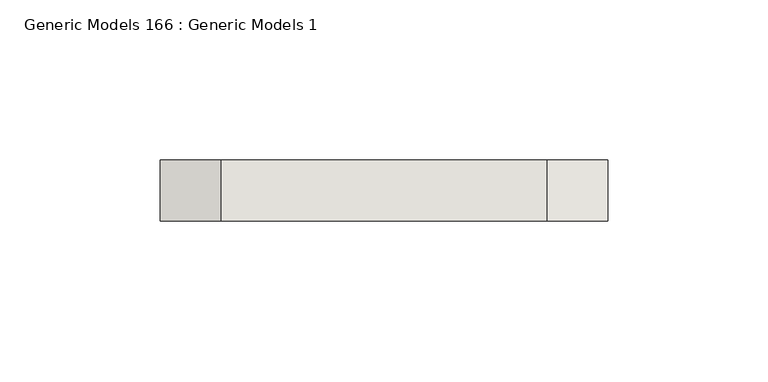
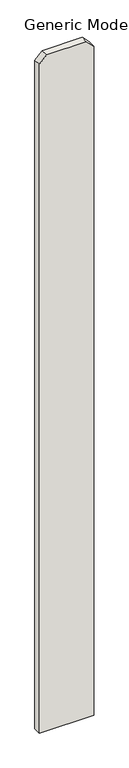
"""IFC4 building model written with IfcOpenShell, lengths in millimetres: wall geometry, Generic Models 166 : Generic Models 1."""

from ifc_helpers import new_model, si_unit, frame, origin, place, context, project, spatial, polyline, outline, extrude, source, transform, mapped, element, save


def generic_models_166_generic_models_1_02abbdc1(model_context):
    return source(origin(), model_context, "Body", "SweptSolid", [
        extrude(outline(polyline([(76.2, 324280.2125), (1885.95, 324280.2125), (1905.0, 324261.1625), (1905.0, 324159.5625), (1885.95, 324140.5125), (76.2, 324140.5125), (76.2, 324280.2125)])), frame((0.0, 547.6875, 0.0), z_axis=(0.0, 1.0, 0.0), x_axis=(0.0, 0.0, 1.0)), (0.0, 0.0, 1.0), 19.05),
    ])


if __name__ == "__main__":
    model = new_model("IFC4")
    model_context = context("Model", 3, world=origin())
    ifc_project = project(units=[si_unit("LENGTHUNIT", "METRE", prefix="MILLI")], contexts=[model_context])
    site = spatial("IfcSite", under=ifc_project)
    building = spatial("IfcBuilding", under=site)
    placement = place(None, origin())
    generic_models_166_generic_models_1_shape = generic_models_166_generic_models_1_02abbdc1(model_context)
    element("IfcWall", 1, ObjectType="Generic Models 166 : Generic Models 1", at=placement, inside=building, context=model_context, shape_type="MappedRepresentation", body=[
        mapped(generic_models_166_generic_models_1_shape, transform((0.0, 0.0, 0.0), x_axis=(1.0, 0.0, 0.0), y_axis=(0.0, 1.0, 0.0), z_axis=(0.0, 0.0, 1.0))),
    ])
    save(model, "model.ifc")

# Revit data of these elements
# Element 1 (IfcWall, "Generic Models 166 : Generic Models 1")
#   Materials on its faces: "VERTICAL 1X6 CEDAR PLANKS W/ CLEAR WOOD SEALER"
# Materials
#   "VERTICAL 1X6 CEDAR PLANKS W/ CLEAR WOOD SEALER": class "Wood", colour RGB 234 198 147, transparency 0, Description = "Pinus Echinata", Cost = 0
